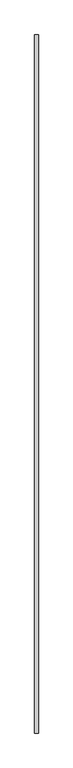
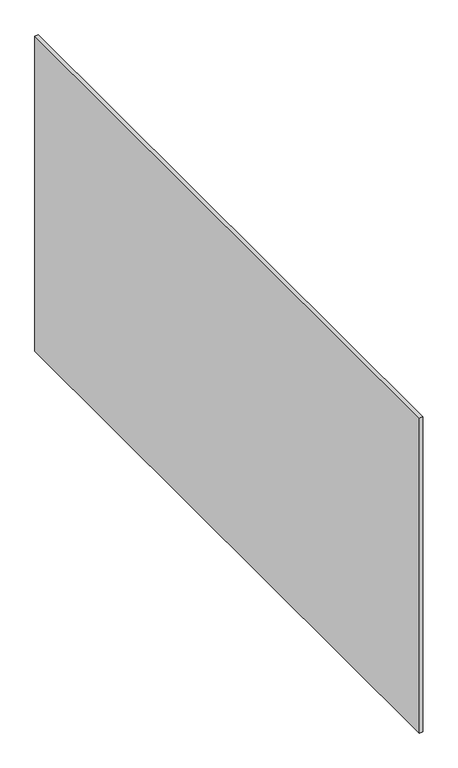
"""IFC4 building model written with IfcOpenShell, lengths in millimetres: proxy geometry, Inner panel:Inner panel:1:Inner panel:1 : Inner panel:Inner panel:300324:300043:Inner panel:1:Inner panel:1 : Inner panel:Inner panel:300324:300043 : Inner panel:Inner panel:1:Inner panel:1 : Inner panel:Inner panel:300324:300043:33 : Inner panel:Inner panel:1:Inner panel:1 : Inner panel:Inner panel:300324:300043:Inner panel:1:Inner panel:1 : Inner panel:Inner panel:300324:300043 : Inner panel:Inner panel:1:Inner panel:1 : Inner panel:Inner panel:300324:300043:300031."""

from ifc_helpers import new_model, si_unit, frame, origin, place, context, project, spatial, polyline, outline, extrude, source, transform, mapped, element, save


def generic_models_50da1861(model_context):
    return source(origin(), model_context, "Body", "SweptSolid", [
        extrude(outline(polyline([(579307.711724, -576279.7163841), (579320.4117239, -576279.7163841), (579320.4117239, -578718.1163841), (579307.711724, -578718.1163841), (579307.711724, -576279.7163841)])), frame((0.0, 0.0, 4946.65), z_axis=(0.0, 0.0, 1.0), x_axis=(1.0, 0.0, 0.0)), (0.0, 0.0, 1.0), 1219.2),
    ])


if __name__ == "__main__":
    model = new_model("IFC4")
    model_context = context("Model", 3, world=origin())
    ifc_project = project(units=[si_unit("LENGTHUNIT", "METRE", prefix="MILLI")], contexts=[model_context])
    site = spatial("IfcSite", under=ifc_project)
    building = spatial("IfcBuilding", under=site)
    placement = place(None, origin())
    generic_models_shape = generic_models_50da1861(model_context)
    element("IfcBuildingElementProxy", 1, Name="Inner panel:Inner panel:1:Inner panel:1 : Inner panel:Inner panel:300324:300043:Inner panel:1:Inner panel:1 : Inner panel:Inner panel:300324:300043 : Inner panel:Inner panel:1:Inner panel:1 : Inner panel:Inner panel:300324:300043:33 : Inner panel:Inner panel:1:Inner panel:1 : Inner panel:Inner panel:300324:300043:Inner panel:1:Inner panel:1 : Inner panel:Inner panel:300324:300043 : Inner panel:Inner panel:1:Inner panel:1 : Inner panel:Inner panel:300324:300043:300031", ObjectType="Inner panel:Inner panel:1:Inner panel:1 : Inner panel:Inner panel:300324:300043:Inner panel:1:Inner panel:1 : Inner panel:Inner panel:300324:300043 : Inner panel:Inner panel:1:Inner panel:1 : Inner panel:Inner panel:300324:300043:33 : Inner panel:Inner panel:1:Inner panel:1 : Inner panel:Inner panel:300324:300043:Inner panel:1:Inner panel:1 : Inner panel:Inner panel:300324:300043 : Inner panel:Inner panel:1:Inner panel:1 : Inner panel:Inner panel:300324:300043:300031", at=placement, inside=building, context=model_context, shape_type="MappedRepresentation", body=[
        mapped(generic_models_shape, transform((0.0, 0.0, 0.0), x_axis=(1.0, 0.0, 0.0), y_axis=(0.0, 1.0, 0.0), z_axis=(0.0, 0.0, 1.0))),
    ])
    save(model, "model.ifc")

# Revit data of these elements
# Type "Inner panel:Inner panel:1:Inner panel:1 : Inner panel:Inner panel:300324:300043:Inner panel:1:Inner panel:1 : Inner panel:Inner panel:300324:300043 : Inner panel:Inner panel:1:Inner panel:1 : Inner panel:Inner panel:300324:300043:33 : Inner panel:Inner panel:1:Inner panel:1 : Inner panel:Inner panel:300324:300043:Inner panel:1:Inner panel:1 : Inner panel:Inner panel:300324:300043 : Inner panel:Inner panel:1:Inner panel:1 : Inner panel:Inner panel:300324:300043:300031"
#   NameOverride = "Inner panel:Inner panel:1:Inner panel:1 : Inner panel:Inner panel:300324:300043:Inner panel:1:Inner panel:1 : Inner panel:Inner panel:300324:300043 : Inner panel:Inner panel:1:Inner panel:1 : Inner panel:Inner panel:300324:300043:300031"
#   ObjectTypeOverride = "Inner panel:1:Inner panel:1 : Inner panel:Inner panel:300324:300043 : Inner panel:Inner panel:1:Inner panel:1 : Inner panel:Inner panel:300324:300043"
#   Reference = "Inner panel"
#   Tag = "300031"
# Element 1 (IfcBuildingElementProxy, "Inner panel:Inner panel:1:Inner panel:1 : Inner panel:Inner panel:300324:300043:Inner panel:1:Inner panel:1 : Inner panel:Inner panel:300324:300043 : Inner panel:Inner panel:1:Inner panel:1 : Inner panel:Inner panel:300324:300043:33 : Inner panel:Inner panel:1:Inner panel:1 : Inner panel:Inner panel:300324:300043:Inner panel:1:Inner panel:1 : Inner panel:Inner panel:300324:300043 : Inner panel:Inner panel:1:Inner panel:1 : Inner panel:Inner panel:300324:300043:300031")
#   Materials on its faces: "1/2\" EXTERIOR GRADE FIRE RETARDANT CDX PLYWOOD"
# Materials
#   "1/2\" EXTERIOR GRADE FIRE RETARDANT CDX PLYWOOD": class "Unassigned", colour RGB 196 177 123, transparency 0, Cost = 0
